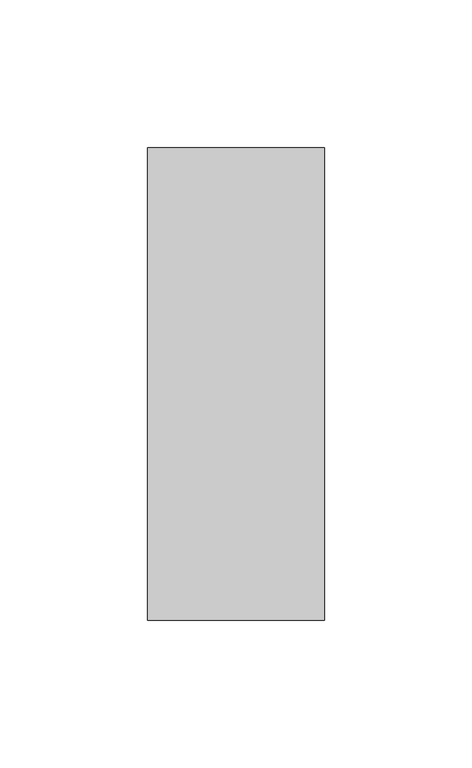
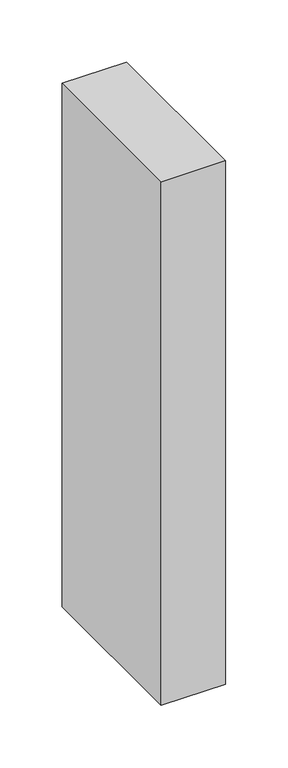
"""IFC4 building model written with IfcOpenShell, lengths in millimetres: column geometry, Madeira de lei-Coluna : Pontalete 6X16cm."""

from ifc_helpers import new_model, si_unit, frame, origin, place, context, project, spatial, polyline, outline, extrude, source, transform, mapped, element, save


def column_e8b88e91(model_context):
    return source(origin(), model_context, "Body", "SweptSolid", [
        extrude(outline(polyline([(30.0, 80.0), (30.0, -80.0), (-30.0, -80.0), (-30.0, 80.0), (30.0, 80.0)])), frame((0.0, 0.0, 6710.0), z_axis=(0.0, 0.0, 1.0), x_axis=(1.0, 0.0, 0.0)), (0.0, 0.0, 1.0), 515.0),
    ])


if __name__ == "__main__":
    model = new_model("IFC4")
    model_context = context("Model", 3, world=origin())
    ifc_project = project(units=[si_unit("LENGTHUNIT", "METRE", prefix="MILLI")], contexts=[model_context])
    site = spatial("IfcSite", under=ifc_project)
    building = spatial("IfcBuilding", under=site)
    placement = place(None, origin())
    column_shape = column_e8b88e91(model_context)
    element("IfcColumn", 1, ObjectType="Madeira de lei-Coluna : Pontalete 6X16cm", at=placement, inside=building, context=model_context, shape_type="MappedRepresentation", body=[
        mapped(column_shape, transform((0.0, 0.0, 0.0), x_axis=(1.0, 0.0, 0.0), y_axis=(0.0, 1.0, 0.0), z_axis=(0.0, 0.0, 1.0))),
    ])
    save(model, "model.ifc")

# Revit data of these elements
# Type "Madeira de lei-Coluna : Pontalete 6X16cm"
#   A = 0.01952 m²
#   b = 0.06 m
#   d = 0.16 m
#   Structural Material [instance default] = none
#   Assembly Code = ""
# Element 1 (IfcColumn, "Madeira de lei-Coluna : Pontalete 6X16cm")
#   Structural Material = .MADEIRAMENTO
#   Materials on its faces: ".MADEIRAMENTO"
# Materials
#   ".MADEIRAMENTO": class ".CC_MADEIRAS", colour RGB 212 179 113, transparency 0, Cost = 0
